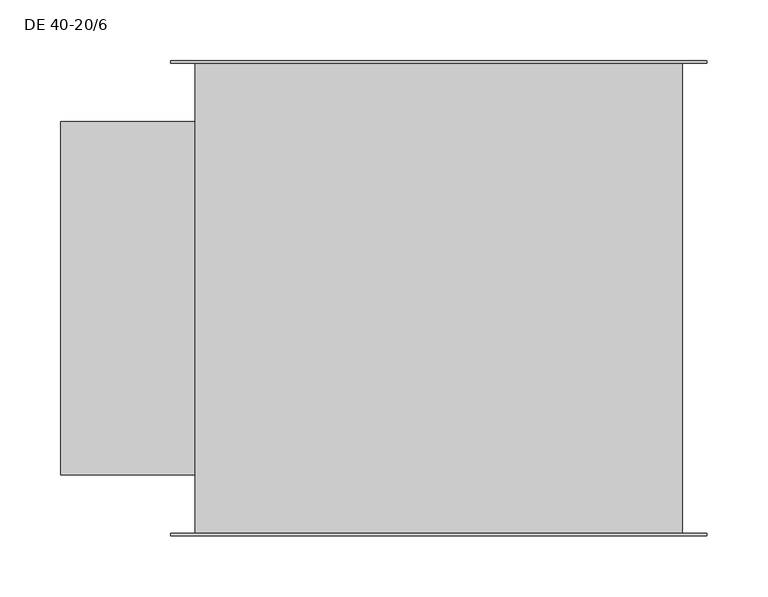
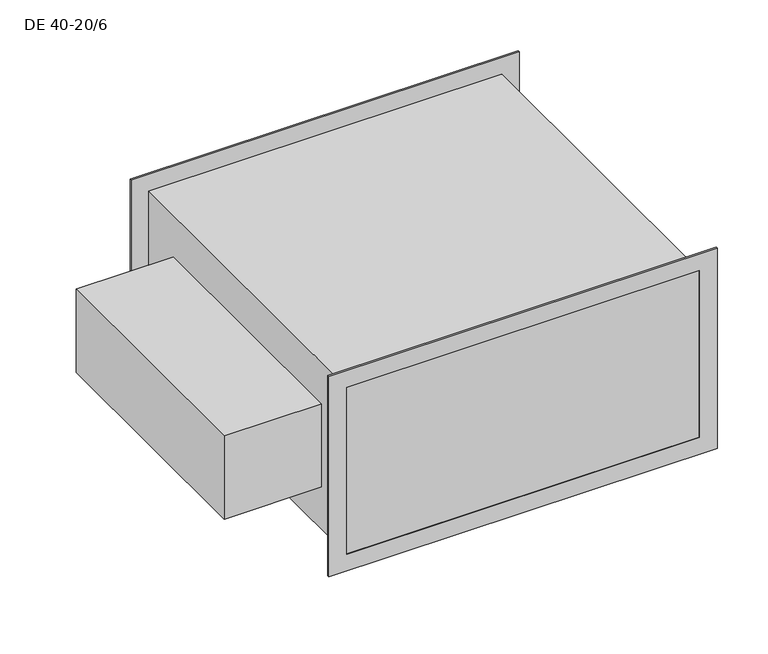
"""IFC4 building model written with IfcOpenShell, lengths in millimetres: proxy geometry, Воздухонагреватель электрический DE : DE 40-20/6."""

import ifcopenshell
import ifcopenshell.guid

model = None  # the IFC model being written
_history = None  # IfcOwnerHistory: only IFC2X3 demands one
_inside = {}  # id of a spatial element -> (the spatial element, [elements in it])
_under = {}  # id of a project, library or spatial element -> (it, [spatial elements below it])
_declared = {}  # id of a project -> (the project, [libraries it declares])
_typed = {}  # id of a type object -> (the type object, [elements of that type])
_made_of = {}  # id of a material, layer set ... -> (it, [elements and type objects made of it])


def new_model(schema):
    """Start an empty IFC model of exactly this schema.

    Asked for "IFC4X3", IfcOpenShell would pick the latest addendum, in which some entities
    have other attributes; the version numbers below select the first issue.
    IFC2X3 requires an IfcOwnerHistory on every rooted entity: one is made here for all.
    """
    global model, _history
    if schema == "IFC4X3":
        model = ifcopenshell.file(schema_version=(4, 3, 0, 0))
    else:
        model = ifcopenshell.file(schema=schema)
    _inside.clear()
    _under.clear()
    _declared.clear()
    _typed.clear()
    _made_of.clear()
    _history = None
    if model.schema == "IFC2X3":
        org = make("IfcOrganization", Name="unknown")
        user = make(
            "IfcPersonAndOrganization",
            ThePerson=make("IfcPerson", FamilyName="unknown"),
            TheOrganization=org,
        )
        app = make(
            "IfcApplication",
            ApplicationDeveloper=org,
            Version="unknown",
            ApplicationFullName="unknown",
            ApplicationIdentifier="unknown",
        )
        _history = make(
            "IfcOwnerHistory",
            OwningUser=user,
            OwningApplication=app,
            ChangeAction="ADDED",
            CreationDate=0,
        )
    return model


def make(cls, **values):
    """One entity of the class cls with the attributes given. An attribute that is None is left unset."""
    return model.create_entity(
        cls, **{name: value for name, value in values.items() if value is not None}
    )


def rooted(cls, **values):
    """An entity with a GlobalId (a new one), such as an element, a storey or a relation."""
    return make(cls, GlobalId=ifcopenshell.guid.new(), OwnerHistory=_history, **values)


def si_unit(unit_type, name, prefix=None):
    """IfcSIUnit, for example si_unit("LENGTHUNIT", "METRE", prefix="MILLI")."""
    return make("IfcSIUnit", UnitType=unit_type, Prefix=prefix, Name=name)


def assignment(units):
    """IfcUnitAssignment: the units of a project."""
    return None if units is None else make("IfcUnitAssignment", Units=units)


def point(xyz):
    """IfcCartesianPoint."""
    return None if xyz is None else make("IfcCartesianPoint", Coordinates=xyz)


def direction(xyz):
    """IfcDirection."""
    return None if xyz is None else make("IfcDirection", DirectionRatios=xyz)


def frame(location, z_axis=None, x_axis=None):
    """IfcAxis2Placement3D, a coordinate frame: its origin and axes. An axis left out is left unset."""
    return make(
        "IfcAxis2Placement3D",
        Location=point(location),
        Axis=direction(z_axis),
        RefDirection=direction(x_axis),
    )


def origin():
    """The frame at (0, 0, 0) with its axes left unset."""
    return frame((0.0, 0.0, 0.0))


def place(relative_to, where):
    """IfcLocalPlacement: puts the frame where relative to a parent placement (None: the world)."""
    return make(
        "IfcLocalPlacement", PlacementRelTo=relative_to, RelativePlacement=where
    )


def context(
    kind, dimensions, precision=None, world=None, true_north=None, identifier=None
):
    """IfcGeometricRepresentationContext, for example the 3D "Model" context."""
    return make(
        "IfcGeometricRepresentationContext",
        ContextIdentifier=identifier,
        ContextType=kind,
        CoordinateSpaceDimension=dimensions,
        Precision=precision,
        WorldCoordinateSystem=world,
        TrueNorth=true_north,
    )


def project(units=None, contexts=None):
    """IfcProject with its units and contexts."""
    return rooted(
        "IfcProject",
        Name="project",
        RepresentationContexts=contexts,
        UnitsInContext=assignment(units),
    )


def spatial(cls, under=None, at=None, **own):
    """A site, building, storey or space (cls), placed at a placement, below another one or the project."""
    s = rooted(cls, ObjectPlacement=at, **own)
    if under is not None:
        _under.setdefault(under.id(), (under, []))[1].append(s)
    return s


def polyline(points):
    """IfcPolyline through the points."""
    return make("IfcPolyline", Points=[point(p) for p in points])


def outline(outer, holes=None, kind="AREA"):
    """IfcArbitraryClosedProfileDef: a profile drawn as a closed curve; with holes, ...WithVoids."""
    if holes is None:
        return make("IfcArbitraryClosedProfileDef", ProfileType=kind, OuterCurve=outer)
    return make(
        "IfcArbitraryProfileDefWithVoids",
        ProfileType=kind,
        OuterCurve=outer,
        InnerCurves=holes,
    )


def extrude(swept, where, along, depth):
    """IfcExtrudedAreaSolid: the profile swept, set in the frame where, extruded along a direction by depth."""
    return make(
        "IfcExtrudedAreaSolid",
        SweptArea=swept,
        Position=where,
        ExtrudedDirection=direction(along),
        Depth=depth,
    )


def shape(context_of_items, identifier, shape_type, items):
    """IfcShapeRepresentation: the items that make up one representation, for example the "Body"."""
    return make(
        "IfcShapeRepresentation",
        ContextOfItems=context_of_items,
        RepresentationIdentifier=identifier,
        RepresentationType=shape_type,
        Items=items,
    )


def source(mapping_origin, context_of_items, identifier, shape_type, items):
    """IfcRepresentationMap: a shape defined once, which mapped items show again and again."""
    return make(
        "IfcRepresentationMap",
        MappingOrigin=mapping_origin,
        MappedRepresentation=shape(context_of_items, identifier, shape_type, items),
    )


def transform(
    local_origin,
    x_axis=None,
    y_axis=None,
    z_axis=None,
    scale=None,
    scale2=None,
    scale3=None,
    uniform=True,
):
    """IfcCartesianTransformationOperator3D, or its non-uniform kind. x_axis, y_axis, z_axis: its Axis1, 2, 3."""
    if uniform:
        return make(
            "IfcCartesianTransformationOperator3D",
            Axis1=direction(x_axis),
            Axis2=direction(y_axis),
            LocalOrigin=point(local_origin),
            Scale=scale,
            Axis3=direction(z_axis),
        )
    return make(
        "IfcCartesianTransformationOperator3DnonUniform",
        Axis1=direction(x_axis),
        Axis2=direction(y_axis),
        LocalOrigin=point(local_origin),
        Scale=scale,
        Axis3=direction(z_axis),
        Scale2=scale2,
        Scale3=scale3,
    )


def mapped(mapping_source, mapping_target):
    """IfcMappedItem: shows the shape of a source again, moved by a transform."""
    return make(
        "IfcMappedItem", MappingSource=mapping_source, MappingTarget=mapping_target
    )


def made_of(thing, what):
    """Note that an element or type object is made of a material, layer set ...; save() writes the relation."""
    if what is not None:
        _made_of.setdefault(what.id(), (what, []))[1].append(thing)
    return thing


def element(
    cls,
    number,
    at=None,
    inside=None,
    cuts=None,
    type_object=None,
    material=None,
    context=None,
    identifier="Body",
    shape_type=None,
    held_by="IfcProductDefinitionShape",
    body=None,
    shapes=None,
    **own,
):
    """One element of the class cls, such as IfcWall. Its Tag is "e" and its number.

    at: its placement. inside: the storey or other place that contains it. cuts: it is an
    opening in that element (IfcRelVoidsElement). A single representation is given by context,
    identifier, shape_type and body (its items); several are given by shapes. held_by: the class
    of the entity that holds the representations. save() writes the other relations.
    """
    e = rooted(cls, Tag="e%d" % number, ObjectPlacement=at, **own)
    if body is not None:
        shapes = [shape(context, identifier, shape_type, body)]
    if shapes is not None:
        e.Representation = make(held_by, Representations=shapes)
    if inside is not None:
        _inside.setdefault(inside.id(), (inside, []))[1].append(e)
    if cuts is not None:
        rooted(
            "IfcRelVoidsElement", RelatingBuildingElement=cuts, RelatedOpeningElement=e
        )
    if type_object is not None:
        _typed.setdefault(type_object.id(), (type_object, []))[1].append(e)
    return made_of(e, material)


def aggregate(whole, parts):
    """IfcRelAggregates: a whole, such as a stair, and the parts it consists of."""
    return rooted("IfcRelAggregates", RelatingObject=whole, RelatedObjects=parts)


def save(model, path):
    """Write the relations noted so far, then the file.

    IfcRelAggregates (storeys below a building ...), IfcRelContainedInSpatialStructure (elements
    in a storey), IfcRelDefinesByType, IfcRelAssociatesMaterial and IfcRelDeclares: one each for
    every whole, place, type object, material and project.
    """
    for whole, parts in _under.values():
        aggregate(whole, parts)
    for where, things in _inside.values():
        rooted(
            "IfcRelContainedInSpatialStructure",
            RelatedElements=things,
            RelatingStructure=where,
        )
    for kind, things in _typed.values():
        rooted("IfcRelDefinesByType", RelatedObjects=things, RelatingType=kind)
    for what, things in _made_of.values():
        rooted("IfcRelAssociatesMaterial", RelatedObjects=things, RelatingMaterial=what)
    for by, libraries in _declared.values():
        rooted("IfcRelDeclares", RelatingContext=by, RelatedDefinitions=libraries)
    model.write(path)


def de_40_20_6_f23ce0ae(model_context):
    return source(origin(), model_context, "Body", "SweptSolid", [
        extrude(outline(polyline([(-200.0, 145.0), (-200.0, -145.0), (-310.0, -145.0), (-310.0, 145.0), (-200.0, 145.0)])), frame((0.0, 0.0, -50.0), z_axis=(0.0, 0.0, 1.0), x_axis=(1.0, 0.0, 0.0)), (0.0, 0.0, 1.0), 100.0),
        extrude(outline(polyline([(120.0, 220.0), (120.0, -220.0), (-120.0, -220.0), (-120.0, 220.0), (120.0, 220.0)]), holes=[polyline([(-100.0, 200.0), (-100.0, -200.0), (100.0, -200.0), (100.0, 200.0), (-100.0, 200.0)])]), frame((0.0, 193.0, 0.0), z_axis=(0.0, 1.0, 0.0), x_axis=(0.0, 0.0, 1.0)), (0.0, 0.0, 1.0), 2.0),
        extrude(outline(polyline([(120.0, -220.0), (-120.0, -220.0), (-120.0, 220.0), (120.0, 220.0), (120.0, -220.0)]), holes=[polyline([(100.0, 200.0), (-100.0, 200.0), (-100.0, -200.0), (100.0, -200.0), (100.0, 200.0)])]), frame((0.0, -195.0, 0.0), z_axis=(0.0, 1.0, 0.0), x_axis=(0.0, 0.0, 1.0)), (0.0, 0.0, 1.0), 2.0),
        extrude(outline(polyline([(200.0, -195.0), (-200.0, -195.0), (-200.0, 195.0), (200.0, 195.0), (200.0, -195.0)])), frame((0.0, 0.0, -100.0), z_axis=(0.0, 0.0, 1.0), x_axis=(1.0, 0.0, 0.0)), (0.0, 0.0, 1.0), 200.0),
    ])


if __name__ == "__main__":
    model = new_model("IFC4")
    model_context = context("Model", 3, world=origin())
    ifc_project = project(units=[si_unit("LENGTHUNIT", "METRE", prefix="MILLI")], contexts=[model_context])
    site = spatial("IfcSite", under=ifc_project)
    building = spatial("IfcBuilding", under=site)
    placement = place(None, origin())
    de_40_20_6_shape = de_40_20_6_f23ce0ae(model_context)
    element("IfcBuildingElementProxy", 1, Name="Воздухонагреватель электрический DE : DE 40-20/6", ObjectType="Воздухонагреватель электрический DE : DE 40-20/6", at=placement, inside=building, context=model_context, shape_type="MappedRepresentation", body=[
        mapped(de_40_20_6_shape, transform((0.0, 0.0, 0.0), x_axis=(1.0, 0.0, 0.0), y_axis=(0.0, 1.0, 0.0), z_axis=(0.0, 0.0, 1.0))),
    ])
    save(model, "model.ifc")

# Revit data of these elements
# Type "Воздухонагреватель электрический DE : DE 40-20/6"
#   Manufacturer = "WAER"
#   URL = "https://waer-air.com/"
#   ADSK_Система_Имя [instance default] = ""
#   ADSK_Наименование краткое = "DE 40-20/6"
#   ADSK_Наименование = "Воздухонагреватель электрический DE 40-20/6"
#   ADSK_Масса_Текст = "9.6"
#   ADSK_Марка = ""
#   ADSK_Код изделия = ""
#   ADSK_Завод-изготовитель = "WAER"
#   ADSK_Единица измерения = "шт."
#   ADSK_Ширина_Б = 510 mm
#   ADSK_Ток = 9.11606 A
#   ADSK_Тепловая мощность = 6000 W
#   ADSK_Расход воздуха = 0 m³/h
#   ADSK_Размер_Ширина = 400 mm
#   ADSK_Размер_Длина_А = 390 mm
#   ADSK_Размер_Высота = 200 mm
#   ADSK_Потеря давления воздуха = 0.0 Pa
#   ADSK_Полная мощность = 6000 VA
#   ADSK_Номинальная мощность = 6000 W
#   ADSK_Напряжение = 380 V
#   ADSK_Масса = 9.6
#   ADSK_Количество ступеней = 1
#   ADSK_Количество = 1
#   ADSK_Количество фаз = 3
#   ADSK_Классификация нагрузок = ОВК
#   Default Elevation = 0
#   Keynote = ""
